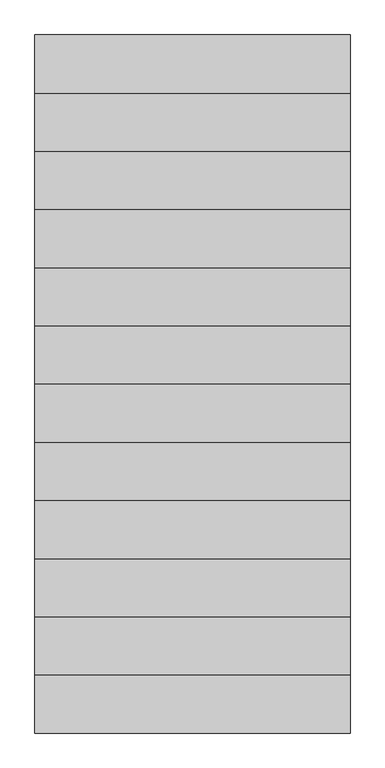
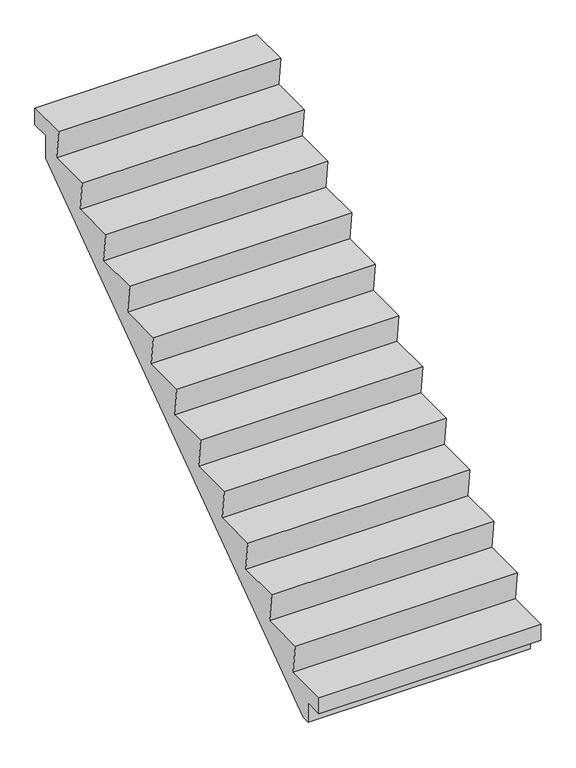
"""IFC4 building model written with IfcOpenShell, lengths in millimetres: proxy geometry, NLRS_24_GM_LB_rechte steektrap prefab-AV_gen_rsf : prefab trap_gen__aant=11 b=1200 a=220 o=172.7 zonder bomen."""

from ifc_helpers import new_model, si_unit, frame, origin, place, context, project, spatial, polyline, outline, extrude, source, transform, mapped, element, save


def generic_models_98d4c19e(model_context):
    return source(origin(), model_context, "Body", "SweptSolid", [
        extrude(outline(polyline([(2400.0, 1900.0), (2640.0, 1900.0), (2640.0, 1800.0), (2530.0, 1800.0), (2530.0, 1658.5925892), (-80.254966, -220.0), (-130.0, -220.0), (-130.0, -100.0), (-240.0, -100.0), (-240.0, 0.0), (20.0, 0.0), (0.0, 172.7272727), (260.0, 172.7272727), (240.0, 345.4545455), (500.0, 345.4545455), (480.0, 518.1818182), (740.0, 518.1818182), (720.0, 690.9090909), (980.0, 690.9090909), (960.0, 863.6363636), (1220.0, 863.6363636), (1200.0, 1036.3636364), (1460.0, 1036.3636364), (1440.0, 1209.0909091), (1700.0, 1209.0909091), (1680.0, 1381.8181818), (1940.0, 1381.8181818), (1920.0, 1554.5454545), (2180.0, 1554.5454545), (2160.0, 1727.2727273), (2420.0, 1727.2727273), (2400.0, 1900.0)])), frame((-650.0, 0.0, 0.0), z_axis=(1.0, 0.0, 0.0), x_axis=(0.0, 1.0, 0.0)), (0.0, 0.0, 1.0), 1300.0),
    ])


if __name__ == "__main__":
    model = new_model("IFC4")
    model_context = context("Model", 3, world=origin())
    ifc_project = project(units=[si_unit("LENGTHUNIT", "METRE", prefix="MILLI")], contexts=[model_context])
    site = spatial("IfcSite", under=ifc_project)
    building = spatial("IfcBuilding", under=site)
    placement = place(None, origin())
    generic_models_shape = generic_models_98d4c19e(model_context)
    element("IfcBuildingElementProxy", 1, Name="NLRS_24_GM_LB_rechte steektrap prefab-AV_gen_rsf : prefab trap_gen__aant=11 b=1200 a=220 o=172.7 zonder bomen", ObjectType="NLRS_24_GM_LB_rechte steektrap prefab-AV_gen_rsf : prefab trap_gen__aant=11 b=1200 a=220 o=172.7 zonder bomen", at=placement, inside=building, context=model_context, shape_type="MappedRepresentation", body=[
        mapped(generic_models_shape, transform((0.0, 0.0, 0.0), x_axis=(1.0, 0.0, 0.0), y_axis=(0.0, 1.0, 0.0), z_axis=(0.0, 0.0, 1.0))),
    ])
    save(model, "model.ifc")

# Revit data of these elements
# Type "NLRS_24_GM_LB_rechte steektrap prefab-AV_gen_rsf : prefab trap_gen__aant=11 b=1200 a=220 o=172.7 zonder bomen"
#   Export Type to IFC As = "IfcStair"
#   Type IfcGUID = "2CEqVLPNH8KRN7ghwV3Z03"
#   Type Comments = " "
#   Model = " "
#   Manufacturer = " "
#   Keynote = " "
#   Description = "rechte steektrap prefab\r\naant=11 b=1200 a=220 o=181,8\r\nzonder bomen"
#   Assembly Code = "24.11"
#   Aantrede onder = 240 mm
#   Width = 1300 mm
#   Wel diepte = 20 mm
#   Trapboom breedte = 0 mm
#   Thickness = 120 mm
#   Optrede onderste trede = 220 mm
#   NLRS_C_lengte = 2400 mm
#   Length = 2880 mm
#   Hoogte oplegnok onder = 100 mm
#   Hoogte oplegnok boven = 100 mm
#   Height = 1900 mm
#   Breedte oplegnok boven = 110 mm
#   BottomCalc = 0 mm
#   Actual Tread Depth = 240 mm
#   Actual Riser Height = 172.727 mm
#   Actual Number of Tread = 10
#   Actual Number of Risers = 11
#   Aantrede boven = 240 mm
#   Aantal treden max dertig = 11
#   Trapboom = no
#   Oplegnok onder = yes
#   NLRS_C_materiaal = NLRS_f2_beton prefab_gen_rsf
#   Default Elevation = 0
# Element 1 (IfcBuildingElementProxy, "NLRS_24_GM_LB_rechte steektrap prefab-AV_gen_rsf : prefab trap_gen__aant=11 b=1200 a=220 o=172.7 zonder bomen")
#   Materials on its faces: "NLRS_f2_beton prefab_gen_rsf"
# Materials
#   "NLRS_f2_beton prefab_gen_rsf": class "F - Niet gebakken kunststeen", colour RGB 129 133 118, transparency 0, Keynote = "f2", Manufacturer = "Revit Standards Foundation", URL = "www.revitstandards.org", Description = "beton prefab", Cost = 0
